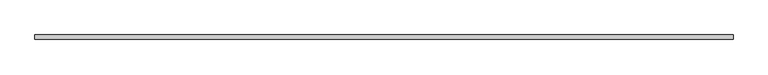
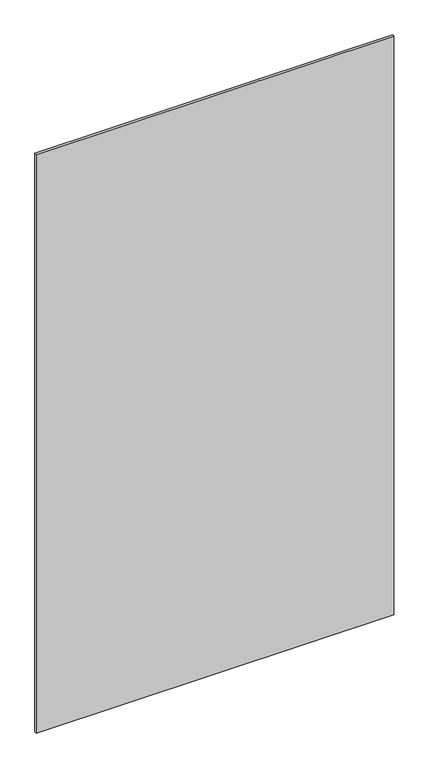
"""IFC4 building model written with IfcOpenShell, lengths in millimetres: proxy geometry, Panel:Panel:300402:Panel:300402 : Panel:Panel:300402:300124:Panel:300402:Panel:300402 : Panel:Panel:300402:300124 : Panel:Panel:300402:Panel:300402 : Panel:Panel:300402:300124:11 : Panel:Panel:300402:Panel:300402 : Panel:Panel:300402:300124:Panel:300402:Panel:300402 : Panel:Panel:300402:300124 : Panel:Panel:300402:Panel:300402 : Panel:Panel:300402:300124:300083."""

from ifc_helpers import new_model, si_unit, frame, origin, place, context, project, spatial, polyline, outline, extrude, source, transform, mapped, element, save


def generic_models_e96d67b6(model_context):
    return source(origin(), model_context, "Body", "SweptSolid", [
        extrude(outline(polyline([(577805.9367239, -579076.8913841), (579025.1367239, -579076.8913841), (579025.1367239, -579084.8288841), (577805.9367239, -579084.8288841), (577805.9367239, -579076.8913841)])), frame((0.0, 0.0, 4049.5374827), z_axis=(0.0, 0.0, 1.0), x_axis=(1.0, 0.0, 0.0)), (0.0, 0.0, 1.0), 2084.5625173),
    ])


if __name__ == "__main__":
    model = new_model("IFC4")
    model_context = context("Model", 3, world=origin())
    ifc_project = project(units=[si_unit("LENGTHUNIT", "METRE", prefix="MILLI")], contexts=[model_context])
    site = spatial("IfcSite", under=ifc_project)
    building = spatial("IfcBuilding", under=site)
    placement = place(None, origin())
    generic_models_shape = generic_models_e96d67b6(model_context)
    element("IfcBuildingElementProxy", 1, Name="Panel:Panel:300402:Panel:300402 : Panel:Panel:300402:300124:Panel:300402:Panel:300402 : Panel:Panel:300402:300124 : Panel:Panel:300402:Panel:300402 : Panel:Panel:300402:300124:11 : Panel:Panel:300402:Panel:300402 : Panel:Panel:300402:300124:Panel:300402:Panel:300402 : Panel:Panel:300402:300124 : Panel:Panel:300402:Panel:300402 : Panel:Panel:300402:300124:300083", ObjectType="Panel:Panel:300402:Panel:300402 : Panel:Panel:300402:300124:Panel:300402:Panel:300402 : Panel:Panel:300402:300124 : Panel:Panel:300402:Panel:300402 : Panel:Panel:300402:300124:11 : Panel:Panel:300402:Panel:300402 : Panel:Panel:300402:300124:Panel:300402:Panel:300402 : Panel:Panel:300402:300124 : Panel:Panel:300402:Panel:300402 : Panel:Panel:300402:300124:300083", at=placement, inside=building, context=model_context, shape_type="MappedRepresentation", body=[
        mapped(generic_models_shape, transform((0.0, 0.0, 0.0), x_axis=(1.0, 0.0, 0.0), y_axis=(0.0, 1.0, 0.0), z_axis=(0.0, 0.0, 1.0))),
    ])
    save(model, "model.ifc")

# Revit data of these elements
# Type "Panel:Panel:300402:Panel:300402 : Panel:Panel:300402:300124:Panel:300402:Panel:300402 : Panel:Panel:300402:300124 : Panel:Panel:300402:Panel:300402 : Panel:Panel:300402:300124:11 : Panel:Panel:300402:Panel:300402 : Panel:Panel:300402:300124:Panel:300402:Panel:300402 : Panel:Panel:300402:300124 : Panel:Panel:300402:Panel:300402 : Panel:Panel:300402:300124:300083"
#   NameOverride = "Panel:Panel:300402:Panel:300402 : Panel:Panel:300402:300124:Panel:300402:Panel:300402 : Panel:Panel:300402:300124 : Panel:Panel:300402:Panel:300402 : Panel:Panel:300402:300124:300083"
#   ObjectTypeOverride = "Panel:300402:Panel:300402 : Panel:Panel:300402:300124 : Panel:Panel:300402:Panel:300402 : Panel:Panel:300402:300124"
#   Reference = "Panel"
#   Tag = "300083"
# Element 1 (IfcBuildingElementProxy, "Panel:Panel:300402:Panel:300402 : Panel:Panel:300402:300124:Panel:300402:Panel:300402 : Panel:Panel:300402:300124 : Panel:Panel:300402:Panel:300402 : Panel:Panel:300402:300124:11 : Panel:Panel:300402:Panel:300402 : Panel:Panel:300402:300124:Panel:300402:Panel:300402 : Panel:Panel:300402:300124 : Panel:Panel:300402:Panel:300402 : Panel:Panel:300402:300124:300083")
#   Materials on its faces: "5/16\" PHENOLIC RESIN PANELS (CLASS A FLAME SPREAD) - EXPOSED FASTENERS"
# Materials
#   "5/16\" PHENOLIC RESIN PANELS (CLASS A FLAME SPREAD) - EXPOSED FASTENERS": class "Unassigned", colour RGB 64 64 64, transparency 0, Keynote = "M07420000.01", Cost = 0
